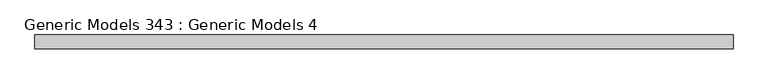
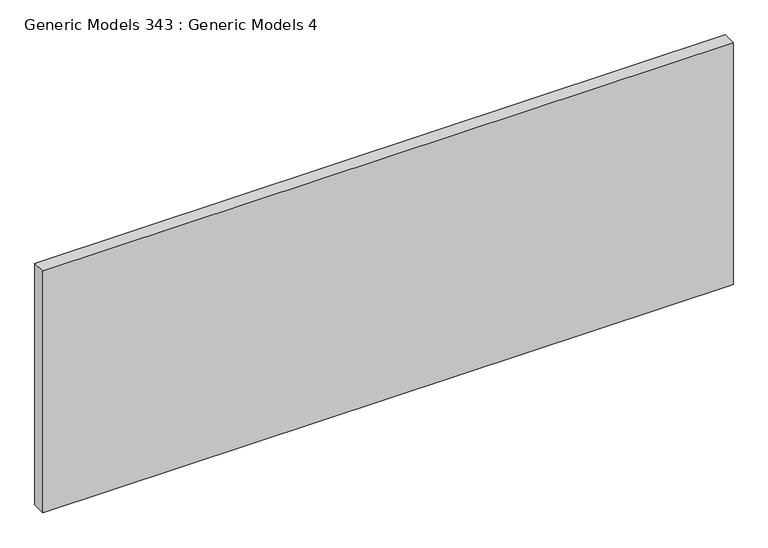
"""IFC4 building model written with IfcOpenShell, lengths in millimetres: proxy geometry, Generic Models 343 : Generic Models 4."""

from ifc_helpers import new_model, si_unit, frame, origin, place, context, project, spatial, polyline, outline, extrude, source, transform, mapped, element, save


def generic_models_343_generic_models_4_691fa667(model_context):
    return source(origin(), model_context, "Body", "SweptSolid", [
        extrude(outline(polyline([(8386.8578684, -6924.2070379), (8386.8578684, -7046.8543523), (2196.9263704, -7046.8543523), (2196.9263704, -6924.2070379), (8386.8578684, -6924.2070379)])), frame((0.0, 0.0, 124104.2281407), z_axis=(0.0, 0.0, 1.0), x_axis=(1.0, 0.0, 0.0)), (0.0, 0.0, 1.0), 2292.0407227),
    ])


if __name__ == "__main__":
    model = new_model("IFC4")
    model_context = context("Model", 3, world=origin())
    ifc_project = project(units=[si_unit("LENGTHUNIT", "METRE", prefix="MILLI")], contexts=[model_context])
    site = spatial("IfcSite", under=ifc_project)
    building = spatial("IfcBuilding", under=site)
    placement = place(None, origin())
    generic_models_343_generic_models_4_shape = generic_models_343_generic_models_4_691fa667(model_context)
    element("IfcBuildingElementProxy", 1, Name="Generic Models 343 : Generic Models 4", ObjectType="Generic Models 343 : Generic Models 4", at=placement, inside=building, context=model_context, shape_type="MappedRepresentation", body=[
        mapped(generic_models_343_generic_models_4_shape, transform((0.0, 0.0, 0.0), x_axis=(1.0, 0.0, 0.0), y_axis=(0.0, 1.0, 0.0), z_axis=(0.0, 0.0, 1.0))),
    ])
    save(model, "model.ifc")

# Revit data of these elements
# Element 1 (IfcBuildingElementProxy, "Generic Models 343 : Generic Models 4")
#   Materials on its faces: "_BATT INSUL. (U-FACTOR = 0.065 MIN.) OVER CLASS II VAPOR RETARDER(TOWARD INTERIOR)"
# Materials
#   "_BATT INSUL. (U-FACTOR = 0.065 MIN.) OVER CLASS II VAPOR RETARDER(TOWARD INTERIOR)": class "Generic", colour RGB 227 210 251, transparency 0, Cost = 0
